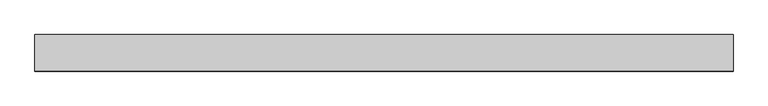
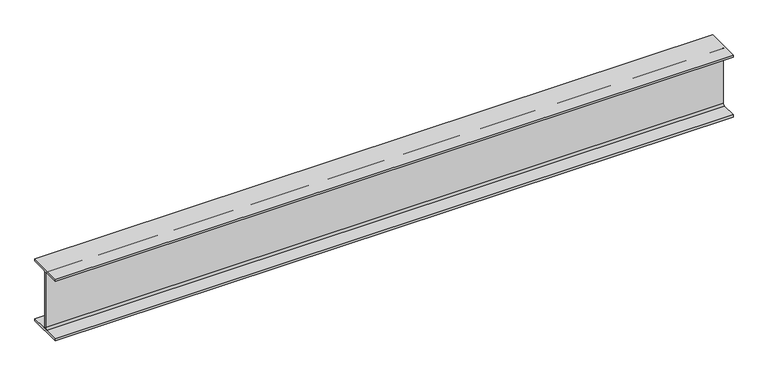
"""IFC4 building model written with IfcOpenShell, lengths in millimetres: beam geometry, Old_Steel Beam_H-KSD3502 : H_SB_ASB_H-250×125x6x9."""

from ifc_helpers import new_model, si_unit, point, frame, frame_2d, origin, place, context, project, spatial, polyline, circle_curve, trimmed, segment, composite_curve, outline, extrude, source, transform, mapped, element, save


def beam_62a9c391(model_context):
    return source(origin(), model_context, "Body", "SweptSolid", [
        extrude(outline(composite_curve([segment(polyline([(82.5, -141.5), (82.5, -151.7), (-82.5, -151.7), (-82.5, -141.5), (-11.9, -141.5)]), True, "CONTINUOUS"), segment(trimmed(circle_curve(frame_2d((-11.9, -132.6)), 8.9), [point((-11.9, -141.5))], [point((-3.0, -132.6))], True, "CARTESIAN"), True, "CONTINUOUS"), segment(polyline([(-3.0, -132.6), (-3.0, 132.6)]), True, "CONTINUOUS"), segment(trimmed(circle_curve(frame_2d((-11.9, 132.6)), 8.9), [point((-3.0, 132.6))], [point((-11.9, 141.5))], True, "CARTESIAN"), True, "CONTINUOUS"), segment(polyline([(-11.9, 141.5), (-82.5, 141.5), (-82.5, 151.7), (82.5, 151.7), (82.5, 141.5), (11.9, 141.5)]), True, "CONTINUOUS"), segment(trimmed(circle_curve(frame_2d((11.9, 132.6)), 8.9), [point((11.9, 141.5))], [point((3.0, 132.6))], True, "CARTESIAN"), True, "CONTINUOUS"), segment(polyline([(3.0, 132.6), (3.0, -132.6)]), True, "CONTINUOUS"), segment(trimmed(circle_curve(frame_2d((11.9, -132.6)), 8.9), [point((3.0, -132.6))], [point((11.9, -141.5))], True, "CARTESIAN"), True, "CONTINUOUS"), segment(polyline([(11.9, -141.5), (82.5, -141.5)]), True, "CONTINUOUS")], self_intersect=False)), frame((-1654.8000435, 0.0, 0.0), z_axis=(1.0, 0.0, 0.0), x_axis=(0.0, 1.0, 0.0)), (0.0, 0.0, 1.0), 3149.2888185),
    ])


if __name__ == "__main__":
    model = new_model("IFC4")
    model_context = context("Model", 3, world=origin())
    ifc_project = project(units=[si_unit("LENGTHUNIT", "METRE", prefix="MILLI")], contexts=[model_context])
    site = spatial("IfcSite", under=ifc_project)
    building = spatial("IfcBuilding", under=site)
    placement = place(None, origin())
    beam_shape = beam_62a9c391(model_context)
    element("IfcBeam", 1, ObjectType="Old_Steel Beam_H-KSD3502 : H_SB_ASB_H-250×125x6x9", at=placement, inside=building, context=model_context, shape_type="MappedRepresentation", body=[
        mapped(beam_shape, transform((0.0, 0.0, 0.0), x_axis=(1.0, 0.0, 0.0), y_axis=(0.0, 1.0, 0.0), z_axis=(0.0, 0.0, 1.0))),
    ])
    save(model, "model.ifc")

# Revit data of these elements
# Type "Old_Steel Beam_H-KSD3502 : H_SB_ASB_H-250×125x6x9"
#   Width = 12.5 cm
#   Web Thickness = 0.6 cm
#   Web Fillet = 1.2 cm
#   Warping Constant = 42539.8 cm⁶
#   Torsional Moment of Inertia = 7.8102 cm⁴
#   Torsional Modulus = 1.0 cm³
#   Section Area = 37.66 cm²
#   Plastic Modulus weak axis = 73.1 cm³
#   Plastic Modulus strong axis = 366.0 cm³
#   Perimeter = 0.97 m²/m
#   Nominal Weight = 29.60 kgf/m
#   Moment of Inertia weak axis = 294.00 cm⁴
#   Moment of Inertia strong axis = 4050.00 cm⁴
#   Height = 25.0 cm
#   Flange Thickness = 0.9 cm
#   Elastic Modulus weak axis = 47.0 cm³
#   Elastic Modulus strong axis = 324.0 cm³
#   Centroid Vertical = 12.5 cm
#   Centroid Horizontal = 6.25 cm
#   Length [instance default] = 1.5240 m
#   Structural Material [instance default] = Steel, 45-345
#   Assembly Code = ""
# Element 1 (IfcBeam, "Old_Steel Beam_H-KSD3502 : H_SB_ASB_H-250×125x6x9")
#   Structural Material = none
# Materials
#   "Steel, 45-345": class "Metal", colour RGB 189 187 185, transparency 0, Description = "Steel 345 MPa", Cost = 0
